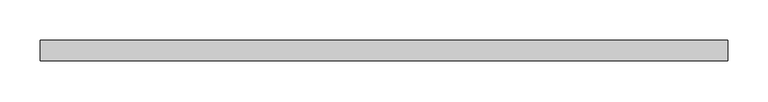
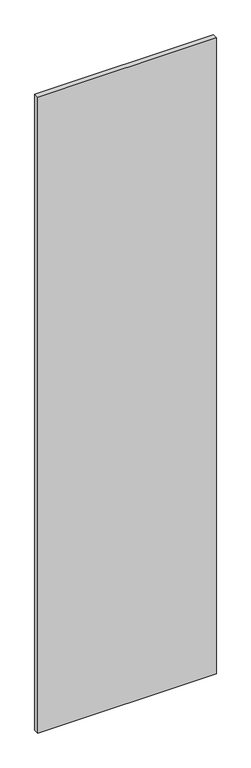
"""IFC4 building model written with IfcOpenShell, lengths in millimetres: plate geometry, 系统嵌板 : 玻璃."""

from ifc_helpers import new_model, si_unit, origin, origin_with_axes, place, context, project, spatial, polyline, outline, extrude, source, transform, mapped, element, save


def plate_d5b4aa06(model_context):
    return source(origin(), model_context, "Body", "SweptSolid", [
        extrude(outline(polyline([(425.0, -12.5), (-425.0, -12.5), (-425.0, 12.5), (425.0, 12.5), (425.0, -12.5)])), origin_with_axes(), (0.0, 0.0, 1.0), 3200.0),
    ])


if __name__ == "__main__":
    model = new_model("IFC4")
    model_context = context("Model", 3, world=origin())
    ifc_project = project(units=[si_unit("LENGTHUNIT", "METRE", prefix="MILLI")], contexts=[model_context])
    site = spatial("IfcSite", under=ifc_project)
    building = spatial("IfcBuilding", under=site)
    placement = place(None, origin())
    plate_shape = plate_d5b4aa06(model_context)
    element("IfcPlate", 1, ObjectType="系统嵌板 : 玻璃", at=placement, inside=building, context=model_context, shape_type="MappedRepresentation", body=[
        mapped(plate_shape, transform((0.0, 0.0, 0.0), x_axis=(1.0, 0.0, 0.0), y_axis=(0.0, 1.0, 0.0), z_axis=(0.0, 0.0, 1.0))),
    ])
    save(model, "model.ifc")

# Revit data of these elements
# Type "系统嵌板 : 玻璃"
#   Construction Type Id = "GSP4R"
#   Analytic Construction = "1/8 英寸 Pilkington 单层玻璃"
#   Visual Light Transmittance = 0.9
#   Solar Heat Gain Coefficient = 0.86
#   Heat Transfer Coefficient (U) = 6.7069 W/(m²·K)
# Element 1 (IfcPlate, "系统嵌板 : 玻璃")
#   Materials on its faces: "玻璃"
# Materials
#   "玻璃": class "玻璃", colour RGB 0 128 192, transparency 0.9, Description = "钠钙玻璃", Cost = 0
